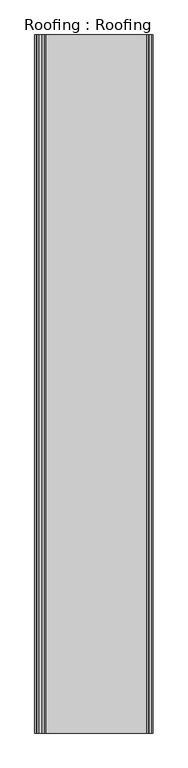
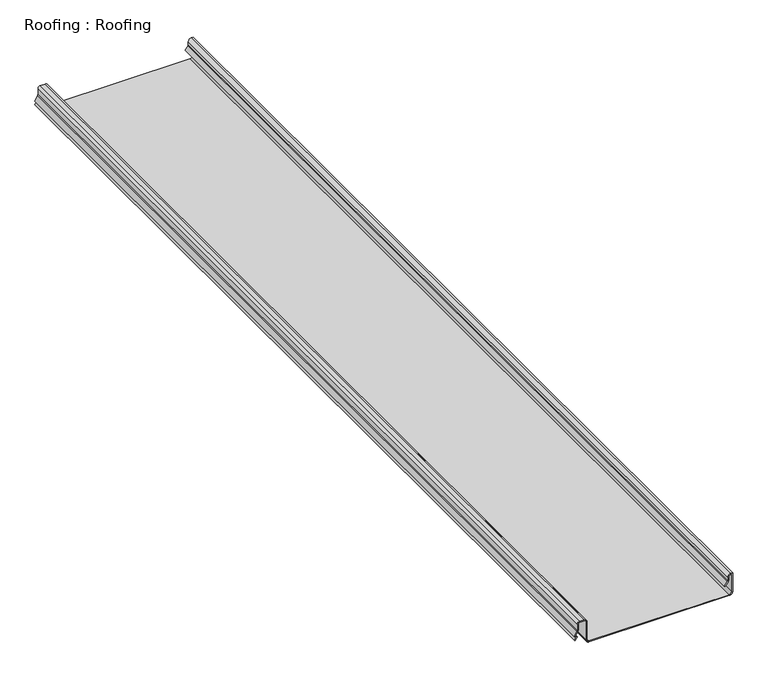
"""IFC4 building model written with IfcOpenShell, lengths in millimetres: proxy geometry, Roofing : Roofing."""

from ifc_helpers import new_model, si_unit, point, frame, frame_2d, origin, place, context, project, spatial, polyline, circle_curve, trimmed, segment, composite_curve, outline, extrude, source, transform, mapped, element, save


def roofing_roofing_e53e7194(model_context):
    return source(origin(), model_context, "Body", "SweptSolid", [
        extrude(outline(composite_curve([segment(trimmed(circle_curve(frame_2d((43490.7540667, -5832.0326367)), 5.08), [point((43487.7710372, -5827.9207108))], [point((43490.7540667, -5826.9526367))], False, "CARTESIAN"), True, "CONTINUOUS"), segment(polyline([(43490.7540667, -5826.9526367), (43497.510625, -5826.9526367)]), True, "CONTINUOUS"), segment(trimmed(circle_curve(frame_2d((43497.510625, -5821.8726367)), 5.08), [point((43497.510625, -5826.9526367))], [point((43502.590625, -5821.8726367))], True, "CARTESIAN"), True, "CONTINUOUS"), segment(polyline([(43502.590625, -5821.8726367), (43502.590625, -5820.277832), (43462.8534375, -5820.277832)]), True, "CONTINUOUS"), segment(trimmed(circle_curve(frame_2d((43462.8534375, -5825.357832)), 5.08), [point((43462.8534375, -5820.277832))], [point((43457.7734375, -5825.357832))], True, "CARTESIAN"), True, "CONTINUOUS"), segment(polyline([(43457.7734375, -5825.357832), (43457.7734375, -6125.6319141)]), True, "CONTINUOUS"), segment(trimmed(circle_curve(frame_2d((43462.8534375, -6125.6319141)), 5.08), [point((43457.7734375, -6125.6319141))], [point((43462.8534375, -6130.7119141))], True, "CARTESIAN"), True, "CONTINUOUS"), segment(polyline([(43462.8534375, -6130.7119141), (43504.466875, -6130.7119141)]), True, "CONTINUOUS"), segment(trimmed(circle_curve(frame_2d((43504.466875, -6135.7919141)), 5.08), [point((43504.466875, -6130.7119141))], [point((43509.546875, -6135.7919141))], False, "CARTESIAN"), True, "CONTINUOUS"), segment(polyline([(43509.546875, -6135.7919141), (43509.546875, -6145.799691)]), True, "CONTINUOUS"), segment(trimmed(circle_curve(frame_2d((43504.466875, -6145.799691)), 5.08), [point((43509.546875, -6145.799691))], [point((43504.466875, -6150.879691))], False, "CARTESIAN"), True, "CONTINUOUS"), segment(polyline([(43504.466875, -6150.879691), (43491.2843008, -6150.879691)]), True, "CONTINUOUS"), segment(trimmed(circle_curve(frame_2d((43491.2843008, -6155.959691)), 5.08), [point((43491.2843008, -6150.879691))], [point((43488.7802894, -6151.5396993))], True, "CARTESIAN"), True, "CONTINUOUS"), segment(polyline([(43488.7802894, -6151.5396993), (43478.2226563, -6157.5208042), (43475.78125, -6153.3567417), (43470.1796875, -6157.3557652), (43469.0176138, -6155.7280107), (43476.399929, -6150.4576863), (43478.9513272, -6154.8093511), (43487.7944581, -6149.7995451)]), True, "CONTINUOUS"), segment(trimmed(circle_curve(frame_2d((43491.2843008, -6155.959691)), 7.08), [point((43487.7944581, -6149.7995451))], [point((43491.2843008, -6148.879691))], False, "CARTESIAN"), True, "CONTINUOUS"), segment(polyline([(43491.2843008, -6148.879691), (43504.466875, -6148.879691)]), True, "CONTINUOUS"), segment(trimmed(circle_curve(frame_2d((43504.466875, -6145.799691)), 3.08), [point((43504.466875, -6148.879691))], [point((43507.546875, -6145.799691))], True, "CARTESIAN"), True, "CONTINUOUS"), segment(polyline([(43507.546875, -6145.799691), (43507.546875, -6135.7919141)]), True, "CONTINUOUS"), segment(trimmed(circle_curve(frame_2d((43504.466875, -6135.7919141)), 3.08), [point((43507.546875, -6135.7919141))], [point((43504.466875, -6132.7119141))], True, "CARTESIAN"), True, "CONTINUOUS"), segment(polyline([(43504.466875, -6132.7119141), (43462.8534375, -6132.7119141)]), True, "CONTINUOUS"), segment(trimmed(circle_curve(frame_2d((43462.8534375, -6125.6319141)), 7.08), [point((43462.8534375, -6132.7119141))], [point((43455.7734375, -6125.6319141))], False, "CARTESIAN"), True, "CONTINUOUS"), segment(polyline([(43455.7734375, -6125.6319141), (43455.7734375, -5825.357832)]), True, "CONTINUOUS"), segment(trimmed(circle_curve(frame_2d((43462.8534375, -5825.357832)), 7.08), [point((43455.7734375, -5825.357832))], [point((43462.8534375, -5818.277832))], False, "CARTESIAN"), True, "CONTINUOUS"), segment(polyline([(43462.8534375, -5818.277832), (43504.590625, -5818.277832), (43504.590625, -5821.8726367)]), True, "CONTINUOUS"), segment(trimmed(circle_curve(frame_2d((43497.510625, -5821.8726367)), 7.08), [point((43504.590625, -5821.8726367))], [point((43497.510625, -5828.9526367))], False, "CARTESIAN"), True, "CONTINUOUS"), segment(polyline([(43497.510625, -5828.9526367), (43490.7540667, -5828.9526367)]), True, "CONTINUOUS"), segment(trimmed(circle_curve(frame_2d((43490.7540667, -5832.0326367)), 3.08), [point((43490.7540667, -5828.9526367))], [point((43488.9454582, -5829.5395793))], True, "CARTESIAN"), True, "CONTINUOUS"), segment(polyline([(43488.9454582, -5829.5395793), (43480.4712961, -5835.6872279), (43479.296875, -5834.0683594), (43487.7710372, -5827.9207108)]), True, "CONTINUOUS")], self_intersect=False)), frame((0.0, 7982.1531721, 0.0), z_axis=(0.0, 1.0, 0.0), x_axis=(0.0, 0.0, 1.0)), (0.0, 0.0, 1.0), 2000.0),
    ])


if __name__ == "__main__":
    model = new_model("IFC4")
    model_context = context("Model", 3, world=origin())
    ifc_project = project(units=[si_unit("LENGTHUNIT", "METRE", prefix="MILLI")], contexts=[model_context])
    site = spatial("IfcSite", under=ifc_project)
    building = spatial("IfcBuilding", under=site)
    placement = place(None, origin())
    roofing_roofing_shape = roofing_roofing_e53e7194(model_context)
    element("IfcBuildingElementProxy", 1, Name="Roofing : Roofing", ObjectType="Roofing : Roofing", at=placement, inside=building, context=model_context, shape_type="MappedRepresentation", body=[
        mapped(roofing_roofing_shape, transform((0.0, 0.0, 0.0), x_axis=(1.0, 0.0, 0.0), y_axis=(0.0, 1.0, 0.0), z_axis=(0.0, 0.0, 1.0))),
    ])
    save(model, "model.ifc")

# Revit data of these elements
# Type "Roofing : Roofing"
#   NameOverride = "Roofing"
# Element 1 (IfcBuildingElementProxy, "Roofing : Roofing")
#   Materials on its faces: "STANDING SEAM METAL ROOF FOLLOW MANU. RECOMMENDED EDGE/TRANSITION DETAILS"
# Materials
#   "STANDING SEAM METAL ROOF FOLLOW MANU. RECOMMENDED EDGE/TRANSITION DETAILS": class "Unassigned", colour RGB 128 128 128, transparency 0, Cost = 0
